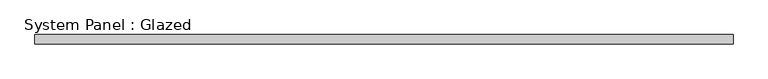
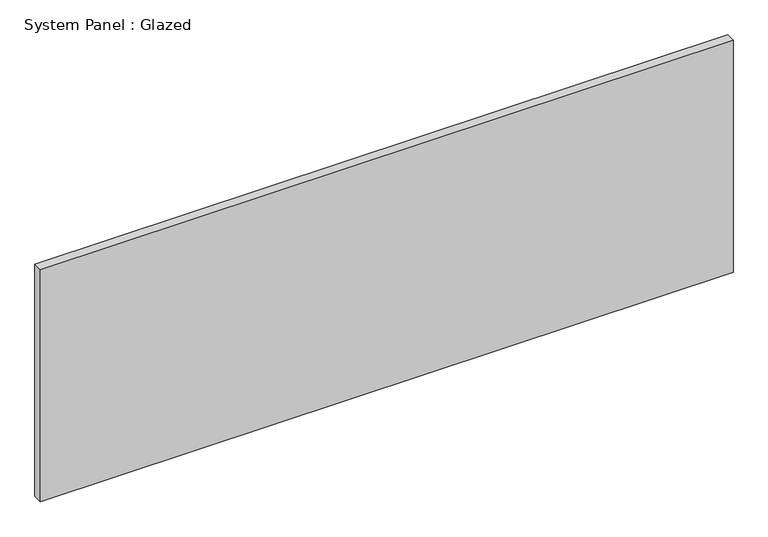
"""IFC4 building model written with IfcOpenShell, lengths in millimetres: plate geometry, System Panel : Glazed."""

from ifc_helpers import new_model, si_unit, origin, origin_with_axes, place, context, project, spatial, polyline, outline, extrude, source, transform, mapped, element, save


def system_panel_glazed_6d97aa7b(model_context):
    return source(origin(), model_context, "Body", "SweptSolid", [
        extrude(outline(polyline([(918.0833333, 24.5), (-918.0833333, 24.5), (-918.0833333, 49.5), (918.0833333, 49.5), (918.0833333, 24.5)])), origin_with_axes(), (0.0, 0.0, 1.0), 650.0),
    ])


if __name__ == "__main__":
    model = new_model("IFC4")
    model_context = context("Model", 3, world=origin())
    ifc_project = project(units=[si_unit("LENGTHUNIT", "METRE", prefix="MILLI")], contexts=[model_context])
    site = spatial("IfcSite", under=ifc_project)
    building = spatial("IfcBuilding", under=site)
    placement = place(None, origin())
    system_panel_glazed_shape = system_panel_glazed_6d97aa7b(model_context)
    element("IfcPlate", 1, ObjectType="System Panel : Glazed", at=placement, inside=building, context=model_context, shape_type="MappedRepresentation", body=[
        mapped(system_panel_glazed_shape, transform((0.0, 0.0, 0.0), x_axis=(1.0, 0.0, 0.0), y_axis=(0.0, 1.0, 0.0), z_axis=(0.0, 0.0, 1.0))),
    ])
    save(model, "model.ifc")

# Revit data of these elements
# Element 1 (IfcPlate, "System Panel : Glazed")
#   Materials on its faces: "Glass"
# Materials
#   "Glass": class "Glass", colour RGB 0 128 192, transparency 0.9
